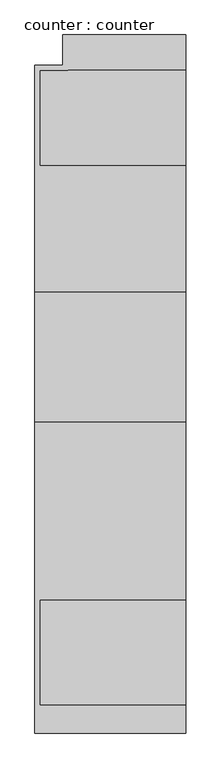
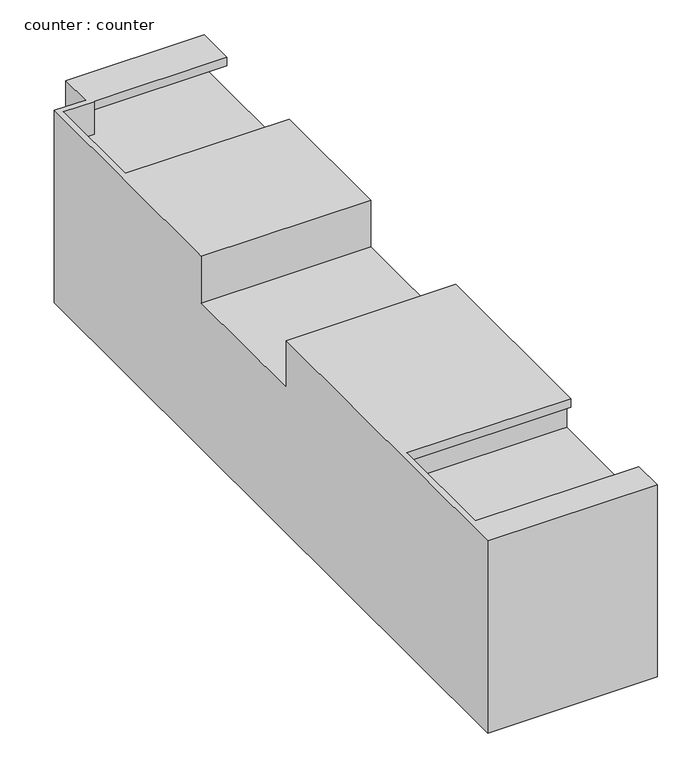
"""IFC4 building model written with IfcOpenShell, lengths in millimetres: furniture geometry, counter : counter."""

from ifc_helpers import new_model, si_unit, origin, place, context, project, spatial, faceted_brep, source, transform, mapped, element, save


def counter_counter_3ed43ffe(model_context):
    return source(origin(), model_context, "Body", "Brep", [
        faceted_brep([(20365.2370052, 2795.2615366, 914.4), (21127.2370052, 2795.2615366, 914.4), (21127.2370052, 2935.6240725, 914.4), (20390.6370052, 2935.6240725, 914.4), (20390.6370052, 3468.3615366, 914.4), (21127.2370052, 3468.3615366, 914.4), (21127.2370052, 4363.7115366, 914.4), (20365.2370052, 4363.7115366, 914.4), (21127.2370052, 6319.5115366, 914.4), (20504.9370052, 6319.5115366, 914.4), (20504.9370052, 6167.1115366, 914.4), (20365.2370052, 6167.1115366, 914.4), (20365.2370052, 5024.1115366, 914.4), (21127.2370052, 5024.1115366, 914.4), (21127.2370052, 5659.1115366, 914.4), (20390.6370052, 5659.1115366, 914.4), (20390.6370052, 6141.7115366, 914.4), (20530.3370052, 6141.7115366, 914.4), (20530.3370052, 6143.8791327, 914.4), (21127.2370052, 6143.8791327, 914.4), (20504.9370052, 6319.5115366, 0.0), (21127.2370052, 6319.5115366, 0.0), (21127.2370052, 6294.1115366, 0.0), (20504.9370052, 6294.1115366, 0.0), (21127.2370052, 2795.2615366, 0.0), (20365.2370052, 2795.2615366, 0.0), (20365.2370052, 6167.1115366, 0.0), (20390.6370052, 6167.1115366, 0.0), (20390.6370052, 5659.1115366, 0.0), (21127.2370052, 5659.1115366, 0.0), (21127.2370052, 5633.7115366, 0.0), (20390.6370052, 5633.7115366, 0.0), (20390.6370052, 5049.5115366, 0.0), (21127.2370052, 5049.5115366, 0.0), (21127.2370052, 4998.7115366, 0.0), (20390.6370052, 4998.7115366, 0.0), (20390.6370052, 4395.4615366, 0.0), (21127.2370052, 4395.4615366, 0.0), (21127.2370052, 4331.9615366, 0.0), (20390.6370052, 4331.9615366, 0.0), (20390.6370052, 3543.7783656, 0.0), (21127.2370052, 3543.7783656, 0.0), (21127.2370052, 3500.1115366, 0.0), (20390.6370052, 3500.1115366, 0.0), (20390.6370052, 2820.9756721, 0.0), (21127.2370052, 2820.9756721, 0.0), (20365.2370052, 4363.7115366, 692.0877523), (20365.2370052, 5024.1115366, 692.0877523), (21127.2370052, 2820.9756721, 86.8174821), (21127.2370052, 3500.1115366, 86.8174821), (21127.2370052, 3543.7783656, 86.8174821), (21127.2370052, 4331.9615366, 86.8174821), (21127.2370052, 4395.4615366, 86.8174821), (21127.2370052, 4998.7115366, 86.8174821), (21127.2370052, 5049.5115366, 86.8174821), (21127.2370052, 5633.7115366, 86.8174821), (21127.2370052, 5659.1115366, 86.8174821), (21127.2370052, 6294.1115366, 86.8174821), (21127.2370052, 6143.8791327, 873.5932433), (21127.2370052, 6294.1115366, 873.5932433), (21127.2370052, 6294.1115366, 758.6706853), (21127.2370052, 5659.1115366, 758.6706853), (21127.2370052, 5024.1115366, 692.0877523), (21127.2370052, 4363.7115366, 692.0877523), (21127.2370052, 3468.3615366, 873.5932433), (21127.2370052, 3500.1115366, 873.5932433), (21127.2370052, 3500.1115366, 758.6706853), (21127.2370052, 2820.9756721, 758.6706853), (21127.2370052, 2820.9756721, 873.5932433), (21127.2370052, 2935.6240725, 873.5932433), (21127.2370052, 5049.5115366, 873.5932433), (21127.2370052, 5621.0115366, 873.5932433), (21127.2370052, 5621.0115366, 591.6951379), (21127.2370052, 5049.5115366, 591.6951379), (21127.2370052, 3543.7783656, 873.5932433), (21127.2370052, 4331.9615366, 873.5932433), (21127.2370052, 4331.9615366, 591.6951379), (21127.2370052, 3543.7783656, 591.6951379), (21127.2370052, 5049.5115366, 555.703506), (21127.2370052, 5621.0115366, 555.703506), (21127.2370052, 5621.0115366, 114.5563816), (21127.2370052, 5049.5115366, 114.5563816), (21127.2370052, 3543.7783656, 555.703506), (21127.2370052, 4331.9615366, 555.703506), (21127.2370052, 4331.9615366, 114.5563816), (21127.2370052, 3543.7783656, 114.5563816), (21127.2370052, 4389.1115366, 555.703506), (21127.2370052, 4998.7115366, 555.703506), (21127.2370052, 4998.7115366, 114.5563816), (21127.2370052, 4389.1115366, 114.5563816), (21127.2370052, 5975.6813885, 726.7328308), (21127.2370052, 6294.1115366, 726.7328308), (21127.2370052, 6294.1115366, 591.6951379), (21127.2370052, 5975.6813885, 591.6951379), (21127.2370052, 5659.1115366, 726.7328308), (21127.2370052, 5951.2115366, 726.7328308), (21127.2370052, 5951.2115366, 591.6951379), (21127.2370052, 5659.1115366, 591.6951379), (21127.2370052, 5659.1115366, 555.703506), (21127.2370052, 6294.1115366, 555.703506), (21127.2370052, 6294.1115366, 114.5563816), (21127.2370052, 5659.1115366, 114.5563816), (21127.2370052, 3169.2590382, 726.7328308), (21127.2370052, 3500.1115366, 726.7328308), (21127.2370052, 3500.1115366, 591.6951379), (21127.2370052, 3169.2590382, 591.6951379), (21127.2370052, 2820.9756721, 726.7328308), (21127.2370052, 3146.9245366, 726.7328308), (21127.2370052, 3146.9245366, 591.6951379), (21127.2370052, 2820.9756721, 591.6951379), (21127.2370052, 2820.9756721, 555.703506), (21127.2370052, 3500.1115366, 555.703506), (21127.2370052, 3500.1115366, 114.5563816), (21127.2370052, 2820.9756721, 114.5563816), (20504.9370052, 6294.1115366, 86.8174821), (20504.9370052, 6167.1115366, 86.8174821), (20504.9370052, 6167.1115366, 114.5563816), (20504.9370052, 6294.1115366, 114.5563816), (20504.9370052, 6294.1115366, 555.703506), (20504.9370052, 6167.1115366, 555.703506), (20504.9370052, 6167.1115366, 591.6951379), (20504.9370052, 6294.1115366, 591.6951379), (20504.9370052, 6294.1115366, 726.7328308), (20504.9370052, 6167.1115366, 726.7328308), (20390.6370052, 6167.1115366, 726.7328308), (20390.6370052, 6167.1115366, 591.6951379), (20390.6370052, 6167.1115366, 555.703506), (20390.6370052, 6167.1115366, 114.5563816), (20390.6370052, 6167.1115366, 86.8174821), (20530.3370052, 6294.1115366, 758.6706853), (20530.3370052, 6141.7115366, 758.6706853), (20390.6370052, 6141.7115366, 758.6706853), (20390.6370052, 5659.1115366, 758.6706853), (20530.3370052, 6294.1115366, 873.5932433), (20530.3370052, 6143.8791327, 873.5932433), (20390.6370052, 5621.0115366, 873.5932433), (20390.6370052, 5049.5115366, 873.5932433), (20390.6370052, 5621.0115366, 591.6951379), (20390.6370052, 5049.5115366, 591.6951379), (20390.6370052, 4331.9615366, 873.5932433), (20390.6370052, 3543.7783656, 873.5932433), (20390.6370052, 4331.9615366, 591.6951379), (20390.6370052, 3543.7783656, 591.6951379), (20390.6370052, 2820.9756721, 873.5932433), (20390.6370052, 2935.6240725, 873.5932433), (20390.6370052, 3500.1115366, 873.5932433), (20390.6370052, 3468.3615366, 873.5932433), (20390.6370052, 3500.1115366, 758.6706853), (20390.6370052, 2820.9756721, 758.6706853), (20390.6370052, 5049.5115366, 555.703506), (20390.6370052, 5621.0115366, 555.703506), (20390.6370052, 5621.0115366, 114.5563816), (20390.6370052, 5049.5115366, 114.5563816), (20390.6370052, 3543.7783656, 555.703506), (20390.6370052, 4331.9615366, 555.703506), (20390.6370052, 4331.9615366, 114.5563816), (20390.6370052, 3543.7783656, 114.5563816), (20390.6370052, 4389.1115366, 555.703506), (20390.6370052, 4998.7115366, 555.703506), (20390.6370052, 4998.7115366, 114.5563816), (20390.6370052, 4389.1115366, 114.5563816), (20390.6370052, 5975.6813885, 726.7328308), (20390.6370052, 5975.6813885, 591.6951379), (20390.6370052, 5659.1115366, 726.7328308), (20390.6370052, 5951.2115366, 726.7328308), (20390.6370052, 5951.2115366, 591.6951379), (20390.6370052, 5659.1115366, 591.6951379), (20390.6370052, 5659.1115366, 555.703506), (20390.6370052, 5659.1115366, 114.5563816), (20390.6370052, 3169.2590382, 726.7328308), (20390.6370052, 3500.1115366, 726.7328308), (20390.6370052, 3500.1115366, 591.6951379), (20390.6370052, 3169.2590382, 591.6951379), (20390.6370052, 2820.9756721, 726.7328308), (20390.6370052, 3146.9245366, 726.7328308), (20390.6370052, 3146.9245366, 591.6951379), (20390.6370052, 2820.9756721, 591.6951379), (20390.6370052, 3543.7783656, 86.8174821), (20390.6370052, 4331.9615366, 86.8174821), (20390.6370052, 4395.4615366, 86.8174821), (20390.6370052, 4998.7115366, 86.8174821), (20390.6370052, 5049.5115366, 86.8174821), (20390.6370052, 5633.7115366, 86.8174821), (20390.6370052, 5659.1115366, 86.8174821), (20390.6370052, 2820.9756721, 86.8174821), (20390.6370052, 3500.1115366, 86.8174821), (20390.6370052, 2820.9756721, 555.703506), (20390.6370052, 3500.1115366, 555.703506), (20390.6370052, 3500.1115366, 114.5563816), (20390.6370052, 2820.9756721, 114.5563816)], [[[0, 1, 2, 3, 4, 5, 6, 7]], [[8, 9, 10, 11, 12, 13, 14, 15, 16, 17, 18, 19]], [[20, 21, 22, 23]], [[24, 25, 26, 27, 28, 29, 30, 31, 32, 33, 34, 35, 36, 37, 38, 39, 40, 41, 42, 43, 44, 45]], [[26, 25, 0, 7, 46, 47, 12, 11]], [[1, 0, 25, 24]], [[1, 24, 45, 48, 49, 42, 41, 50, 51, 38, 37, 52, 53, 34, 33, 54, 55, 30, 29, 56, 57, 22, 21, 8, 19, 58, 59, 60, 61, 14, 13, 62, 63, 6, 5, 64, 65, 66, 67, 68, 69, 2], [70, 71, 72, 73], [74, 75, 76, 77], [78, 79, 80, 81], [82, 83, 84, 85], [86, 87, 88, 89], [90, 91, 92, 93], [94, 95, 96, 97], [98, 99, 100, 101], [102, 103, 104, 105], [106, 107, 108, 109], [110, 111, 112, 113]], [[9, 8, 21, 20]], [[10, 9, 20, 23, 114, 115, 116, 117, 118, 119, 120, 121, 122, 123]], [[11, 10, 123, 124, 125, 120, 119, 126, 127, 116, 115, 128, 27, 26]], [[47, 62, 13, 12]], [[63, 46, 7, 6]], [[62, 47, 46, 63]], [[129, 130, 131, 132, 61, 60]], [[130, 129, 133, 134, 18, 17]], [[131, 130, 17, 16]], [[132, 131, 16, 15]], [[61, 132, 15, 14]], [[59, 133, 129, 60]], [[135, 71, 70, 136]], [[137, 138, 73, 72]], [[135, 136, 138, 137]], [[136, 70, 73, 138]], [[71, 135, 137, 72]], [[133, 59, 58, 134]], [[139, 75, 74, 140]], [[141, 142, 77, 76]], [[139, 140, 142, 141]], [[140, 74, 77, 142]], [[75, 139, 141, 76]], [[68, 143, 144, 69]], [[145, 65, 64, 146]], [[66, 147, 148, 67]], [[65, 145, 147, 66]], [[148, 147, 145, 146, 4, 3, 144, 143]], [[143, 68, 67, 148]], [[78, 149, 150, 79]], [[80, 151, 152, 81]], [[79, 150, 151, 80]], [[150, 149, 152, 151]], [[149, 78, 81, 152]], [[82, 153, 154, 83]], [[84, 155, 156, 85]], [[83, 154, 155, 84]], [[154, 153, 156, 155]], [[153, 82, 85, 156]], [[86, 157, 158, 87]], [[88, 159, 160, 89]], [[87, 158, 159, 88]], [[158, 157, 160, 159]], [[157, 86, 89, 160]], [[90, 161, 124, 123, 122, 91]], [[162, 93, 92, 121, 120, 125]], [[91, 122, 121, 92]], [[161, 162, 125, 124]], [[161, 90, 93, 162]], [[94, 163, 164, 95]], [[96, 165, 166, 97]], [[95, 164, 165, 96]], [[164, 163, 166, 165]], [[163, 94, 97, 166]], [[98, 167, 126, 119, 118, 99]], [[168, 101, 100, 117, 116, 127]], [[99, 118, 117, 100]], [[167, 168, 127, 126]], [[167, 98, 101, 168]], [[102, 169, 170, 103]], [[104, 171, 172, 105]], [[103, 170, 171, 104]], [[170, 169, 172, 171]], [[169, 102, 105, 172]], [[106, 173, 174, 107]], [[108, 175, 176, 109]], [[107, 174, 175, 108]], [[174, 173, 176, 175]], [[173, 106, 109, 176]], [[50, 177, 178, 51]], [[51, 178, 39, 38]], [[178, 177, 40, 39]], [[177, 50, 41, 40]], [[52, 179, 180, 53]], [[53, 180, 35, 34]], [[180, 179, 36, 35]], [[179, 52, 37, 36]], [[54, 181, 182, 55]], [[55, 182, 31, 30]], [[182, 181, 32, 31]], [[181, 54, 33, 32]], [[56, 183, 128, 115, 114, 57]], [[57, 114, 23, 22]], [[183, 28, 27, 128]], [[183, 56, 29, 28]], [[48, 184, 185, 49]], [[49, 185, 43, 42]], [[185, 184, 44, 43]], [[184, 48, 45, 44]], [[110, 186, 187, 111]], [[112, 188, 189, 113]], [[111, 187, 188, 112]], [[187, 186, 189, 188]], [[186, 110, 113, 189]], [[4, 146, 64, 5]], [[144, 3, 2, 69]], [[18, 134, 58, 19]]]),
    ])


if __name__ == "__main__":
    model = new_model("IFC4")
    model_context = context("Model", 3, world=origin())
    ifc_project = project(units=[si_unit("LENGTHUNIT", "METRE", prefix="MILLI")], contexts=[model_context])
    site = spatial("IfcSite", under=ifc_project)
    building = spatial("IfcBuilding", under=site)
    placement = place(None, origin())
    counter_counter_shape = counter_counter_3ed43ffe(model_context)
    element("IfcFurniture", 1, ObjectType="counter : counter", at=placement, inside=building, context=model_context, shape_type="MappedRepresentation", body=[
        mapped(counter_counter_shape, transform((0.0, 0.0, 0.0), x_axis=(1.0, 0.0, 0.0), y_axis=(0.0, 1.0, 0.0), z_axis=(0.0, 0.0, 1.0))),
    ])
    save(model, "model.ifc")

# Revit data of these elements
# Element 1 (IfcFurniture, "counter : counter")
#   Materials on its faces: "food"
# Materials
#   "food": class "Glass", colour RGB 233 233 233, transparency 0, Description = "Soda Lime Glass", Cost = 0
